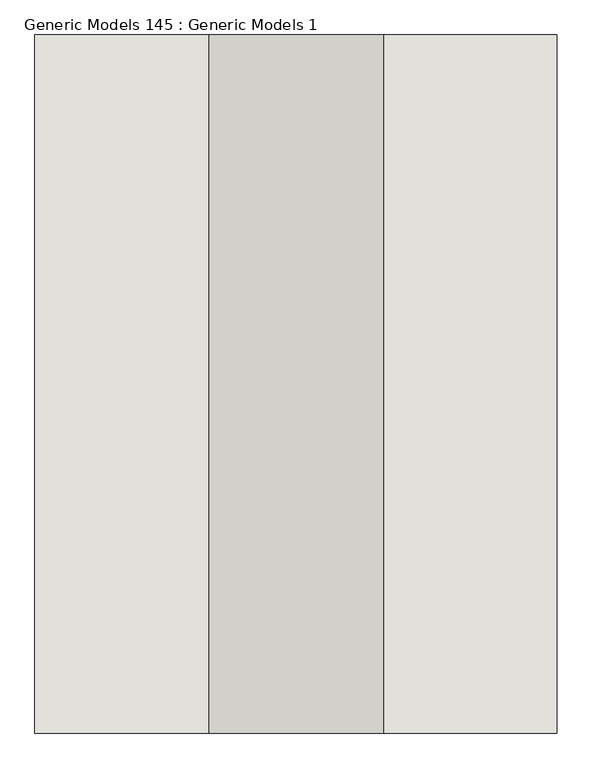
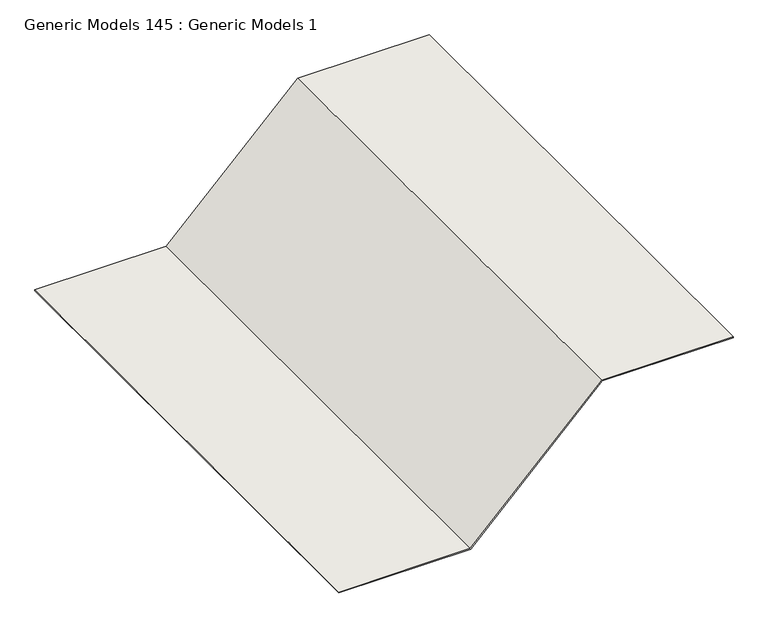
"""IFC4 building model written with IfcOpenShell, lengths in millimetres: wall geometry, Generic Models 145 : Generic Models 1."""

from ifc_helpers import new_model, si_unit, frame, origin, place, context, project, spatial, polyline, outline, extrude, source, transform, mapped, element, save


def generic_models_145_generic_models_1_d1ee8326(model_context):
    return source(origin(), model_context, "Body", "SweptSolid", [
        extrude(outline(polyline([(-155.575, 52785.9625), (-153.9875, 52785.9625), (-153.9875, 52482.353125), (-458.7875, 52177.553125), (-458.7875, 51873.410689), (-460.375, 51873.410689), (-460.375, 52178.210689), (-155.575, 52483.010689), (-155.575, 52785.9625)])), frame((0.0, 0.0, 0.0), z_axis=(0.0, 1.0, 0.0), x_axis=(0.0, 0.0, 1.0)), (0.0, 0.0, 1.0), 1219.2),
    ])


if __name__ == "__main__":
    model = new_model("IFC4")
    model_context = context("Model", 3, world=origin())
    ifc_project = project(units=[si_unit("LENGTHUNIT", "METRE", prefix="MILLI")], contexts=[model_context])
    site = spatial("IfcSite", under=ifc_project)
    building = spatial("IfcBuilding", under=site)
    placement = place(None, origin())
    generic_models_145_generic_models_1_shape = generic_models_145_generic_models_1_d1ee8326(model_context)
    element("IfcWall", 1, ObjectType="Generic Models 145 : Generic Models 1", at=placement, inside=building, context=model_context, shape_type="MappedRepresentation", body=[
        mapped(generic_models_145_generic_models_1_shape, transform((0.0, 0.0, 0.0), x_axis=(1.0, 0.0, 0.0), y_axis=(0.0, 1.0, 0.0), z_axis=(0.0, 0.0, 1.0))),
    ])
    save(model, "model.ifc")

# Revit data of these elements
# Element 1 (IfcWall, "Generic Models 145 : Generic Models 1")
#   Materials on its faces: "6 MIL VAPOR BARRIER"
# Materials
#   "6 MIL VAPOR BARRIER": class "Generic", colour RGB 66 158 52, transparency 0, Cost = 0
